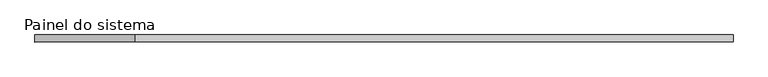
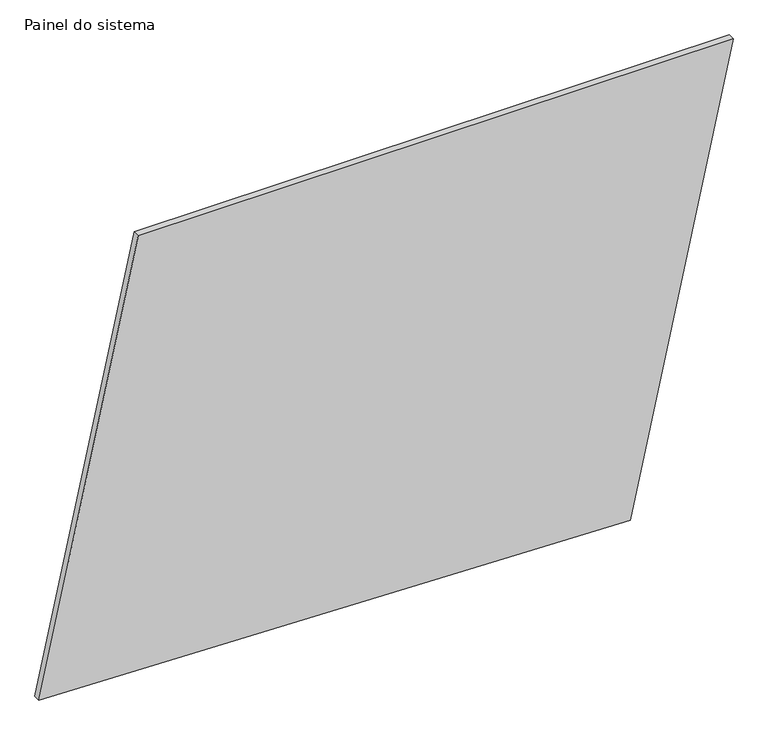
"""IFC4 building model written with IfcOpenShell, lengths in millimetres: plate geometry, Painel do sistema : Envidraçado."""

from ifc_helpers import new_model, si_unit, frame, origin, place, context, project, spatial, polyline, outline, extrude, source, transform, mapped, element, save


def painel_do_sistema_e6263762(model_context):
    return source(origin(), model_context, "Body", "SweptSolid", [
        extrude(outline(polyline([(58.2185789, -1230.7803718), (0.0, 866.5442473), (1676.1490174, 1230.7803718), (1676.1490174, -879.1954551), (58.2185789, -1230.7803718)])), frame((0.0, 24.5, 0.0), z_axis=(0.0, 1.0, 0.0), x_axis=(0.0, 0.0, 1.0)), (0.0, 0.0, 1.0), 25.0),
    ])


if __name__ == "__main__":
    model = new_model("IFC4")
    model_context = context("Model", 3, world=origin())
    ifc_project = project(units=[si_unit("LENGTHUNIT", "METRE", prefix="MILLI")], contexts=[model_context])
    site = spatial("IfcSite", under=ifc_project)
    building = spatial("IfcBuilding", under=site)
    placement = place(None, origin())
    painel_do_sistema_shape = painel_do_sistema_e6263762(model_context)
    element("IfcPlate", 1, ObjectType="Painel do sistema : Envidraçado", at=placement, inside=building, context=model_context, shape_type="MappedRepresentation", body=[
        mapped(painel_do_sistema_shape, transform((0.0, 0.0, 0.0), x_axis=(1.0, 0.0, 0.0), y_axis=(0.0, 1.0, 0.0), z_axis=(0.0, 0.0, 1.0))),
    ])
    save(model, "model.ifc")

# Revit data of these elements
# Type "Painel do sistema : Envidraçado"
#   Construction Type Id = "GSP4R"
#   Analytic Construction = "Vidraça única Pilkington 1/8 pol"
#   Visual Light Transmittance = 0.9
#   Solar Heat Gain Coefficient = 0.86
#   Heat Transfer Coefficient (U) = 6.7069 W/(m²·K)
# Element 1 (IfcPlate, "Painel do sistema : Envidraçado")
#   Materials on its faces: "Vidro"
# Materials
#   "Vidro": class "Vidro", colour RGB 0 128 192, transparency 0.9, Description = "Vidro de sílica", Cost = 0
